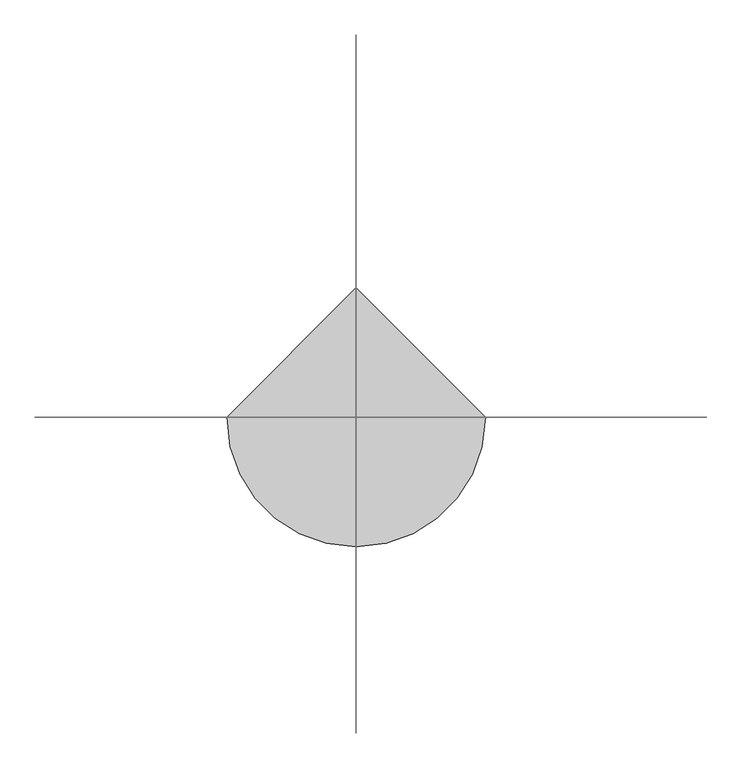
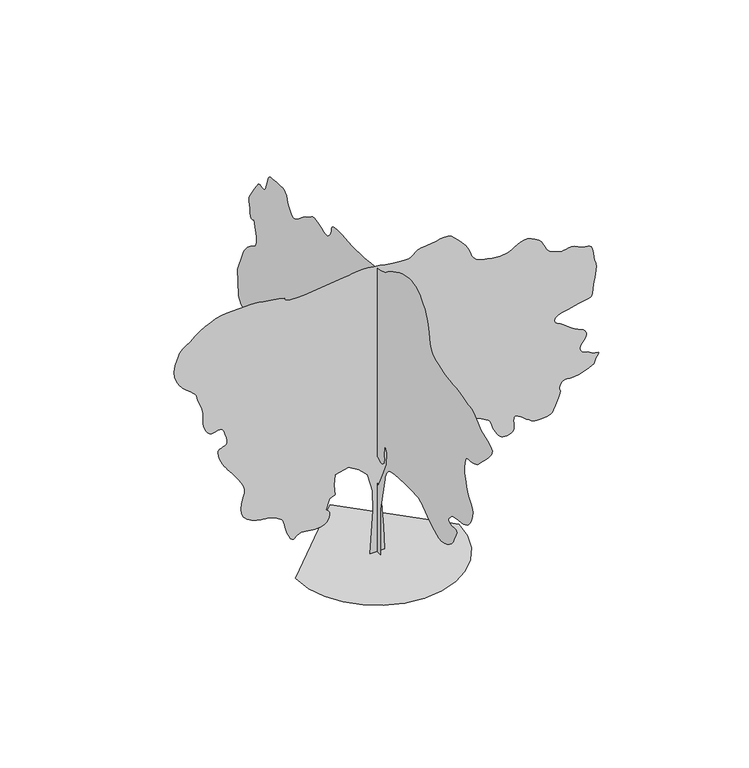
"""IFC4 building model written with IfcOpenShell, lengths in millimetres: geographic element geometry, RPC 木 - 落葉樹 : リンゴの木 - 6.0 メートル."""

from ifc_helpers import new_model, si_unit, origin, place, context, project, spatial, triangles, source, transform, mapped, element, save


def geographic_element_a7a636f8(model_context):
    return source(origin(), model_context, "Body", "Tessellation", [
        triangles([(-6.51e-05, -105.0228319, 0.0074776), (-6.15e-05, 138.9131143, 0.0074703), (-4.84e-05, 99.8833291, 458.6078719), (-3.14e-05, 129.1556067, 1014.7807915), (-1.8e-05, 226.7299288, 1414.8361691), (-8.5e-06, 392.6053236, 1649.0138809), (-1.1e-06, 577.9979682, 1805.1340027), (2.6e-06, 753.6305981, 1844.161417), (3.5e-06, 948.7807503, 1775.8613708), (1.5e-06, 1007.3257959, 1678.2863674), (-4e-06, 890.2357046, 1551.4387321), (-8.4e-06, 929.2657351, 1385.5635372), (-1.44e-05, 1153.685903, 1073.3258371), (-1.47e-05, 1543.9836639, 868.4182137), (-8.5e-06, 2109.9142365, 790.3606236), (7.6e-06, 2451.4244957, 1161.1408985), (2.53e-05, 2802.702182, 1580.7112186), (3.2e-05, 3349.1025513, 1531.9237896), (3.84e-05, 3544.2528488, 1649.0138809), (4.53e-05, 3534.5028625, 1883.1914474), (4.5e-05, 3358.8778267, 1961.2515083), (4.95e-05, 3232.0277206, 2175.9142776), (5.43e-05, 3534.5028625, 2185.6716763), (5.98e-05, 4139.453437, 2068.584201), (6.19e-05, 4208.0283211, 2104.1717091), (6.39e-05, 4273.9283684, 2140.0141434), (6.59e-05, 4334.553447, 2176.3691917), (6.78e-05, 4387.2284294, 2213.4942513), (6.96e-05, 4429.328476, 2251.6417774), (7.12e-05, 4458.2034576, 2291.0693127), (7.26e-05, 4471.2035362, 2332.0343994), (8.79e-05, 4500.4784935, 2829.6522812), (9.79e-05, 4334.6034439, 3249.2275429), (9.86e-05, 4317.5033249, 3282.3275574), (9.94e-05, 4292.2284142, 3321.5527794), (0.0001002, 4260.1033401, 3364.7027618), (0.000101, 4222.5283081, 3409.5526405), (0.0001017, 4180.8532356, 3453.9028404), (0.0001023, 4136.4533295, 3495.527916), (0.0001027, 4090.6782166, 3532.2027122), (0.0001029, 4046.5782921, 3560.9279938), (0.0001029, 4006.7531067, 3582.8278198), (0.000103, 3971.8782005, 3601.8278229), (0.0001031, 3942.6282417, 3621.8527634), (0.0001036, 3919.7031876, 3646.8529816), (0.0001043, 3903.7779968, 3680.7029503), (0.0001056, 3895.5282097, 3727.3530098), (0.0001072, 3894.4779831, 3782.2781456), (0.0001089, 3899.0529945, 3838.2279282), (0.0001108, 3908.3280098, 3895.0532387), (0.0001127, 3921.3530869, 3952.5282188), (0.0001147, 3937.2032822, 4010.528167), (0.0001167, 3954.9280724, 4068.8783844), (0.0001187, 3973.5780968, 4127.4033005), (0.0001184, 3998.5533165, 4107.2783661), (0.0001184, 4022.8532867, 4091.9531387), (0.0001185, 4045.7783409, 4086.1782005), (0.0001191, 4066.6532295, 4094.7532585), (0.0001202, 4084.8032845, 4122.4283134), (0.0001219, 4099.5532562, 4174.003363), (0.0001245, 4110.1781891, 4254.2534065), (0.000127, 4120.6784203, 4333.2285278), (0.0001287, 4132.0283089, 4385.4035408), (0.0001299, 4139.1281662, 4422.2036201), (0.0001309, 4136.8033081, 4455.0786484), (0.0001318, 4120.0031708, 4495.478508), (0.0001331, 4083.5533607, 4554.8286644), (0.0001348, 4022.3783157, 4644.5537109), (0.0001367, 3956.5782623, 4741.1289207), (0.0001382, 3906.9780922, 4815.003772), (0.0001392, 3869.5280525, 4868.5789902), (0.0001398, 3840.0781059, 4904.2041412), (0.0001401, 3814.5529198, 4924.3290756), (0.0001399, 3788.8780334, 4931.3042313), (0.0001393, 3758.9281174, 4927.5038818), (0.0001386, 3727.67799, 4918.0288788), (0.0001379, 3700.2029228, 4909.0788437), (0.0001374, 3675.45298, 4904.7291092), (0.0001372, 3652.4029335, 4909.0788437), (0.0001374, 3630.0528442, 4926.2289597), (0.000138, 3607.3527763, 4960.2792068), (0.0001393, 3583.2777924, 5015.3287537), (0.0001409, 3562.2279144, 5079.6288986), (0.0001424, 3546.3027237, 5137.7538391), (0.0001437, 3531.0527824, 5188.4042358), (0.0001447, 3512.0527794, 5230.1540131), (0.0001452, 3484.8526955, 5261.6794144), (0.0001452, 3445.0278008, 5281.604361), (0.0001446, 3388.1277855, 5288.5295197), (0.0001436, 3319.3276245, 5291.5793335), (0.0001428, 3248.6275795, 5298.5544891), (0.000142, 3178.9774704, 5306.2040222), (0.0001411, 3113.2274139, 5311.3042923), (0.0001402, 3054.3025223, 5310.5793365), (0.0001392, 3005.1273262, 5300.8293503), (0.000138, 2968.5772316, 5278.778952), (0.0001369, 2944.7272339, 5253.1543533), (0.0001361, 2929.602285, 5232.6294434), (0.0001354, 2919.9272942, 5214.0044174), (0.0001347, 2912.4774582, 5194.003894), (0.0001338, 2904.0023941, 5169.4042328), (0.0001326, 2891.2523003, 5136.9288895), (0.000131, 2871.0023735, 5093.3792221), (0.0001292, 2844.6522377, 5045.379245), (0.0001275, 2815.5772682, 5003.1539154), (0.000126, 2783.4271957, 4968.9542587), (0.0001248, 2747.8773308, 4945.0039764), (0.0001238, 2708.5521149, 4933.504097), (0.0001233, 2665.1521477, 4936.7039017), (0.0001232, 2617.3021614, 4956.7788391), (0.0001234, 2569.6771614, 4988.2542435), (0.0001238, 2525.4769524, 5023.3038483), (0.0001243, 2482.1194244, 5060.7288895), (0.0001247, 2437.0593842, 5099.3538574), (0.0001252, 2387.7318718, 5138.0038239), (0.0001254, 2331.5768692, 5175.4288651), (0.0001255, 2266.0343582, 5210.4790512), (0.0001256, 2205.0142456, 5244.5542969), (0.0001259, 2159.0142918, 5277.6040237), (0.0001262, 2120.3541515, 5306.2290207), (0.0001262, 2081.3542065, 5327.0044968), (0.0001258, 2034.3291698, 5336.5044983), (0.0001247, 1971.6040741, 5331.3292328), (0.0001227, 1885.4940685, 5308.0544907), (0.0001205, 1797.391452, 5276.8540695), (0.0001188, 1730.2863911, 5251.9544266), (0.0001175, 1678.8813892, 5236.1042313), (0.0001168, 1637.8888332, 5232.0288986), (0.0001166, 1602.0163136, 5242.4794235), (0.0001169, 1565.9737461, 5270.1544785), (0.0001177, 1524.4687214, 5317.8044769), (0.0001188, 1490.9861721, 5373.8045471), (0.0001201, 1475.2561729, 5423.9793915), (0.0001212, 1466.3511932, 5467.3296524), (0.0001221, 1453.3511147, 5502.8292297), (0.0001225, 1425.3286972, 5529.4543488), (0.0001222, 1371.366148, 5546.1794907), (0.000121, 1280.5334656, 5551.979718), (0.0001195, 1182.4759335, 5550.8792038), (0.0001183, 1108.9958982, 5547.8793869), (0.0001174, 1052.4133781, 5543.5296524), (0.0001165, 1005.0483187, 5538.3293884), (0.0001156, 959.220738, 5532.7791458), (0.0001147, 907.2482563, 5527.4044739), (0.0001136, 841.4482029, 5522.7041794), (0.0001125, 772.3506037, 5519.7043625), (0.0001115, 711.6155754, 5518.9044113), (0.0001107, 653.2705175, 5520.154335), (0.0001099, 591.3404677, 5523.2791443), (0.000109, 519.8504273, 5528.1294296), (0.0001078, 432.8303392, 5534.5046219), (0.0001065, 324.3052774, 5542.2291504), (0.000105, 203.687658, 5552.8796631), (0.0001037, 86.9965703, 5567.6043457), (0.0001026, -21.8426915, 5585.7544006), (0.0001018, -118.9050968, 5606.6292892), (0.0001012, -200.2644113, 5629.5546341), (0.0001011, -261.9952181, 5653.8543137), (0.0001012, -300.1702317, 5678.8295334), (0.0001016, -342.4727732, 5713.0297714), (0.000102, -413.9603428, 5761.2297363), (0.0001023, -506.7854181, 5817.0798157), (0.0001024, -613.0929554, 5874.3298096), (0.0001023, -725.0330704, 5926.6045258), (0.0001019, -834.75319, 5967.6299286), (0.0001011, -934.4057556, 5991.07966), (0.0001, -1022.9033335, 5999.8047089), (9.88e-05, -1104.7484104, 6000.0046967), (9.74e-05, -1180.4459702, 5990.3047073), (9.57e-05, -1250.5110249, 5969.3298248), (9.38e-05, -1315.4560432, 5935.7295502), (9.14e-05, -1375.7936394, 5888.1545471), (8.87e-05, -1432.0336658, 5825.2049011), (8.63e-05, -1478.7161362, 5768.8048553), (8.48e-05, -1512.7687088, 5733.7546692), (8.36e-05, -1538.2837212, 5707.9295013), (8.25e-05, -1559.3636845, 5679.2045105), (8.09e-05, -1580.1012268, 5635.454274), (7.84e-05, -1604.5962433, 5564.5545319), (7.46e-05, -1636.941362, 5454.4042786), (7.05e-05, -1667.1512913, 5330.3292938), (6.7e-05, -1688.656374, 5223.97939), (6.39e-05, -1710.6739254, 5132.8541382), (6.11e-05, -1742.4214062, 5054.3292801), (5.83e-05, -1793.1164223, 4985.8788071), (5.53e-05, -1871.9714928, 4924.9540375), (5.19e-05, -1988.2065491, 4868.9789658), (4.87e-05, -2119.0091755, 4825.5040031), (4.62e-05, -2237.6917568, 4799.6038399), (4.41e-05, -2347.6668755, 4784.9788605), (4.22e-05, -2452.3543808, 4775.3288681), (4.04e-05, -2555.1521759, 4764.2786705), (3.83e-05, -2659.5022018, 4745.5539413), (3.57e-05, -2768.8022163, 4712.8539024), (3.33e-05, -2866.4523605, 4683.5786545), (3.19e-05, -2939.5522591, 4672.2287659), (3.09e-05, -2996.927536, 4668.05373), (2.99e-05, -3047.4773575, 4660.2786232), (2.85e-05, -3100.0773445, 4638.1788094), (2.61e-05, -3163.6025368, 4590.9787834), (2.24e-05, -3246.9276833, 4507.9536186), (1.83e-05, -3354.9527756, 4422.0536293), (1.48e-05, -3474.4277504, 4364.503363), (1.18e-05, -3586.9278603, 4321.8033531), (9.3e-06, -3673.9780701, 4280.47855), (7e-06, -3717.153051, 4227.0283241), (5e-06, -3698.0280556, 4147.9782074), (2.9e-06, -3598.177755, 4029.8281517), (1.1e-06, -3473.4528099, 3906.2781349), (-3e-07, -3385.2276718, 3815.6781418), (-1.3e-06, -3323.4776619, 3751.5279877), (-1.9e-06, -3278.1025246, 3707.3530678), (-2.2e-06, -3239.0275841, 3676.6529068), (-2.3e-06, -3196.2275803, 3652.9528999), (-2.1e-06, -3139.5775497, 3629.777861), (-1.7e-06, -3075.1774109, 3613.37799), (-9e-07, -3016.2275208, 3608.6029907), (-2e-07, -2963.4272552, 3606.7278145), (2e-07, -2917.4774437, 3599.0529922), (2e-07, -2879.0021759, 3576.8528938), (-7e-07, -2848.7272797, 3531.452758), (-2.7e-06, -2827.3521309, 3454.1278267), (-5.1e-06, -2815.7522575, 3369.9277336), (-7e-06, -2813.3521133, 3305.0276253), (-8.6e-06, -2818.6523712, 3252.4026398), (-1.02e-05, -2830.0772552, 3205.052623), (-1.19e-05, -2846.1271477, 3156.0024193), (-1.39e-05, -2865.2274353, 3098.2524559), (-1.64e-05, -2885.9023361, 3024.8022881), (-1.92e-05, -2914.627327, 2946.6774055), (-2.18e-05, -2954.4522217, 2877.5772629), (-2.43e-05, -2998.5524368, 2814.6273262), (-2.67e-05, -3040.0775185, 2754.9021927), (-2.9e-05, -3072.2275909, 2695.5270378), (-3.11e-05, -3088.152491, 2633.6020386), (-3.3e-05, -3081.052343, 2566.2020828), (-3.46e-05, -3060.4274391, 2500.277037), (-3.6e-05, -3039.1022873, 2443.7194427), (-3.71e-05, -3015.2522896, 2395.18694), (-3.79e-05, -2986.9272743, 2353.3118797), (-3.85e-05, -2952.3273514, 2316.7293743), (-3.88e-05, -2909.5023491, 2284.0717747), (-3.89e-05, -2856.6273788, 2253.9743385), (-3.87e-05, -2791.7272705, 2230.5618141), (-3.8e-05, -2717.452153, 2216.0268002), (-3.71e-05, -2638.7520149, 2206.0967377), (-3.62e-05, -2560.5271385, 2196.5117123), (-3.56e-05, -2487.799601, 2182.9993103), (-3.53e-05, -2425.47201, 2161.2942398), (-3.56e-05, -2378.5043827, 2127.129174), (-3.62e-05, -2345.7043499, 2089.8041267), (-3.68e-05, -2322.8042942, 2060.3341232), (-3.73e-05, -2310.1443111, 2037.0066227), (-3.78e-05, -2308.0692924, 2018.1191128), (-3.84e-05, -2316.9168629, 2001.9616688), (-3.92e-05, -2337.029298, 1986.8265461), (-4.01e-05, -2368.7468388, 1971.0090523), (-4.1e-05, -2411.2468609, 1962.5040482), (-4.16e-05, -2459.0394379, 1965.0915356), (-4.21e-05, -2505.4770103, 1970.754126), (-4.27e-05, -2543.876992, 1971.4641117), (-4.34e-05, -2567.6019974, 1959.2041042), (-4.44e-05, -2569.9771431, 1925.949012), (-4.59e-05, -2544.3769615, 1863.6765049), (-4.75e-05, -2509.7520401, 1792.5014889), (-4.89e-05, -2484.8695473, 1735.1513557), (-4.99e-05, -2462.7095627, 1687.5312973), (-5.08e-05, -2436.2819607, 1645.5437439), (-5.14e-05, -2398.5893486, 1605.0912712), (-5.19e-05, -2342.631863, 1562.0787804), (-5.22e-05, -2261.4142914, 1512.4087017), (-5.2e-05, -2169.1316975, 1473.3237328), (-5.1e-05, -2083.5066914, 1461.3762062), (-4.95e-05, -2002.8290577, 1471.4462311), (-4.76e-05, -1925.3965748, 1498.4137711), (-4.53e-05, -1849.4990273, 1537.1587898), (-4.28e-05, -1773.4289612, 1582.5612511), (-4.02e-05, -1695.4838642, 1629.498793), (-3.77e-05, -1622.0062271, 1676.8063705), (-3.54e-05, -1558.0836754, 1724.7963192), (-3.31e-05, -1500.136195, 1770.5689613), (-3.11e-05, -1444.578685, 1811.2214218), (-2.93e-05, -1387.8260445, 1843.8489361), (-2.77e-05, -1326.2960793, 1865.5564774), (-2.64e-05, -1256.4010723, 1873.4340488), (-2.5e-05, -1159.1384045, 1874.2889385), (-2.3e-05, -1027.910804, 1875.4840691), (-2.07e-05, -877.7382116, 1874.971455), (-1.86e-05, -723.6380974, 1870.7039829), (-1.67e-05, -580.6329818, 1860.6339581), (-1.55e-05, -463.7428782, 1842.7115055), (-1.52e-05, -387.9878002, 1814.8914013), (-1.57e-05, -343.2127716, 1776.8839828), (-1.66e-05, -308.1652379, 1730.6863667), (-1.77e-05, -281.2252217, 1677.6614056), (-1.92e-05, -260.7727092, 1619.1738419), (-2.08e-05, -245.1829449, 1556.5887085), (-2.26e-05, -232.8366782, 1491.2736546), (-2.44e-05, -222.1121693, 1424.5935677), (-3.85e-05, -114.7803395, 897.6907001), (-2.01e-05, -26.9632706, 1297.7460777), (-1.3e-05, -173.3248856, 1609.9838505), (-6.5e-06, -300.1727388, 1892.9489914), (2e-07, -319.6852469, 2127.129174), (4.7e-06, -251.3852008, 2244.2167946), (-4e-07, -222.1119331, 2058.8266571), (-1.7e-06, -228.0859325, 2017.1790539), (-3e-06, -232.2679447, 1976.5565334), (-4.1e-06, -232.865183, 1937.9815624), (-5.1e-06, -228.0859325, 1902.4790783), (-5.9e-06, -216.1379155, 1871.0740185), (-6.4e-06, -195.2293988, 1844.788995), (-6.5e-06, -163.5673779, 1824.6489452), (-6.1e-06, -127.1833524, 1819.4714996), (-5.2e-06, -93.5303284, 1831.0189053), (-4.2e-06, -62.949051, 1849.7389835), (-3.3e-06, -35.7820297, 1866.0664753), (-2.9e-06, -12.3698845, 1870.4490566), (-3.1e-06, 6.9458055, 1853.3239391), (-4.3e-06, 21.8237678, 1805.1340027), (-6.1e-06, 32.3777748, 1741.0688725), (-7.7e-06, 39.3472803, 1682.1263947), (-9.3e-06, 43.330036, 1627.4512436), (-1.08e-05, 44.9230347, 1576.1888203), (-1.22e-05, 44.724037, 1527.4862698), (-1.37e-05, 43.330036, 1480.4911732), (-1.51e-05, 41.3385332, 1434.3511116), (137.391859, 0.0003253, 0.0), (-133.3141101, 0.0003334, 0.0), (-73.1573078, 0.0002372, 832.1731876), (-83.1833128, 0.0002433, 1223.1935062), (-183.4456522, 0.0001982, 1574.1087147), (-333.8377625, 0.0002049, 1724.5014244), (-534.3604428, 0.0002126, 1844.8164642), (-785.015601, 0.0002192, 1784.6589443), (-805.0681561, 0.0002168, 1584.1363003), (-785.015601, 0.0002134, 1393.6386257), (-885.278231, 0.0002156, 1343.5060753), (-955.4607931, 0.0002149, 1153.0084007), (-936.3432827, 0.0002675, 1139.8859459), (-918.5407356, 0.0002668, 1125.3558735), (-903.3707314, 0.0002661, 1108.0233559), (-892.1456898, 0.0002654, 1086.4808481), (-886.1831903, 0.0002648, 1059.3258196), (-886.7981964, 0.0002643, 1025.1533415), (-895.3032005, 0.0002639, 982.565752), (-913.9532249, 0.0002639, 940.0632591), (-942.5982788, 0.0002642, 906.5057144), (-978.963283, 0.0002649, 881.0181713), (-1020.7633478, 0.0002659, 862.7181982), (-1065.71838, 0.0002671, 850.7331739), (-1111.553373, 0.0002683, 844.1856812), (-1155.9834372, 0.0002696, 842.1981571), (-1199.4784567, 0.000271, 844.8881819), (-1243.6759769, 0.0002724, 851.4356747), (-1288.0485592, 0.0002738, 859.5631582), (-1332.0685467, 0.0002752, 866.9856703), (-1375.2135876, 0.0002766, 871.4282043), (-1416.9560978, 0.0002778, 870.610667), (-1456.7686386, 0.0002789, 862.2507122), (-1490.9986713, 0.0002796, 844.3906832), (-1518.2137253, 0.0002801, 821.2681847), (-1541.2187164, 0.0002805, 799.9006662), (-1562.8187061, 0.0002809, 787.3031067), (-1585.8236973, 0.0002817, 790.4881594), (-1613.0387512, 0.0002829, 816.475672), (-1647.2663132, 0.0002313, 872.2782251), (-1679.7413658, 0.0002334, 944.3882858), (-1702.0463997, 0.0002351, 1013.3457773), (-1717.508828, 0.0002365, 1077.2133905), (-1729.4639122, 0.0002377, 1134.0684231), (-1741.2438618, 0.0002387, 1181.9784348), (-1756.1814674, 0.0002397, 1219.0134562), (-1777.6064678, 0.0002407, 1243.2460613), (-1804.2939377, 0.0002418, 1262.5659576), (-1833.963929, 0.000243, 1284.8709915), (-1868.368951, 0.0002444, 1308.2261066), (-1909.2639839, 0.000246, 1330.7035137), (-1958.3990662, 0.0002477, 1350.3761501), (-2017.5341194, 0.0002497, 1365.3136105), (-2088.4191822, 0.0002519, 1373.5860706), (-2170.7616852, 0.0002011, 1382.5010788), (-2258.5417923, 0.000204, 1401.9385551), (-2344.9193687, 0.0002071, 1433.8310852), (-2423.054425, 0.0002101, 1480.1036968), (-2486.1043556, 0.0002129, 1542.6862141), (-2527.2271362, 0.0002153, 1623.5087517), (-2539.6019623, 0.0002172, 1724.5014244), (-2528.5270569, 0.0002183, 1822.2489464), (-2508.6771057, 0.0002189, 1897.5490013), (-2487.2420769, 0.0002192, 1958.6416386), (-2471.4293793, 0.0001661, 2013.7690876), (-2468.4170631, 0.0001669, 2071.1791008), (-2485.3994568, 0.0001684, 2139.1117275), (-2529.5769928, 0.000171, 2225.8093426), (-2588.3771828, 0.0001741, 2318.6767845), (-2644.0269836, 0.000177, 2400.3194756), (-2695.8270195, 0.0001796, 2471.7869156), (-2743.0773331, 0.000182, 2534.1270058), (-2785.0520966, 0.0001306, 2588.4271797), (-2821.0522247, 0.0001324, 2635.6772026), (-2850.4021774, 0.0001339, 2676.9770073), (-2878.5522034, 0.0001354, 2723.8270546), (-2908.6274025, 0.0001372, 2782.7522369), (-2936.4274498, 0.000139, 2847.4523575), (-2957.7523109, 0.0001406, 2911.6522179), (-2968.3522453, 0.0001418, 2969.0024963), (-2964.0525078, 0.0001423, 3013.2024147), (-2940.6524826, 0.000142, 3037.927359), (-2905.0023331, 0.0001411, 3050.052491), (-2869.2021927, 0.0001402, 3062.5523094), (-2836.72714, 0.0001395, 3078.1775185), (-2811.1022507, 0.000139, 3099.7773628), (-2795.8023125, 0.000139, 3130.1525436), (-2794.3771088, 0.0001396, 3172.1025993), (-2810.3022995, 0.0001409, 3228.4276497), (-2831.7271545, 8.9e-05, 3286.3526024), (-2846.6774048, 9.02e-05, 3332.2027107), (-2858.4522675, 9.1e-05, 3367.3276016), (-2870.4024101, 9.18e-05, 3393.1777679), (-2885.8523392, 9.25e-05, 3411.1278351), (-2908.17743, 9.33e-05, 3422.5777176), (-2940.6524826, 9.44e-05, 3428.9526192), (-2978.7524826, 9.55e-05, 3427.0527351), (-3016.0025345, 9.65e-05, 3417.4277412), (-3052.7023293, 9.74e-05, 3407.1277885), (-3089.2524239, 9.85e-05, 3403.1027435), (-3125.9775078, 9.97e-05, 3412.4277557), (-3163.2025612, 0.0001012, 3442.1026886), (-3201.3275597, 0.0001032, 3499.1276962), (-3229.5025841, 0.0001051, 3569.6277534), (-3241.3777313, 0.0001065, 3637.1529922), (-3243.9525742, 0.0001076, 3704.8529297), (-3244.2275574, 0.0001086, 3775.9029533), (-3249.2525414, 5.65e-05, 3853.4031647), (-3266.0276802, 5.83e-05, 3940.5780762), (-3301.5775452, 6.09e-05, 4040.5533691), (-3337.877655, 6.33e-05, 4130.928376), (-3357.5276184, 6.48e-05, 4192.7283829), (-3368.4028267, 6.58e-05, 4234.1784691), (-3378.4027977, 6.65e-05, 4263.5284218), (-3395.4276306, 6.74e-05, 4289.0033203), (-3427.3277184, 6.88e-05, 4318.8785316), (-3482.0528664, 7.1e-05, 4361.3785538), (-3552.8529053, 2.06e-05, 4417.8785934), (-3623.6529442, 2.37e-05, 4484.3786041), (-3688.3030678, 2.68e-05, 4561.0535751), (-3740.6780685, 2.96e-05, 4648.0787865), (-3774.6530296, 3.21e-05, 4745.6289368), (-3784.0780357, 3.4e-05, 4853.8540169), (-3762.7778824, 3.51e-05, 4972.9790131), (-3729.8778557, -1.77e-05, 5076.7040771), (-3704.502951, -1.74e-05, 5145.8539261), (-3680.7029503, -1.74e-05, 5191.3290573), (-3652.5279259, -1.78e-05, 5224.0043884), (-3614.0029518, -1.85e-05, 5254.7792542), (-3559.1778099, -1.95e-05, 5294.454158), (-3482.0528664, -2.09e-05, 5353.9790131), (-3391.1775993, -2.26e-05, 5424.8793365), (-3298.9027084, -2.44e-05, 5490.3794083), (-3205.0276245, -2.63e-05, 5548.6543396), (-3109.4273552, -2.84e-05, 5598.0042343), (-3011.8774956, -3.07e-05, 5636.6297836), (-2912.2274734, -3.33e-05, 5662.8293472), (-2810.3022995, -3.62e-05, 5674.8047791), (-2339.0719059, -5.01e-05, 5684.8297485), (-2273.3618179, -5.21e-05, 5682.2043274), (-2197.6542297, -5.44e-05, 5674.854776), (-2113.614156, -3.7e-06, 5663.5293045), (-2022.9115528, -6.6e-06, 5649.0546066), (-1927.2115803, -9.7e-06, 5632.2294708), (-1828.1764915, -1.3e-05, 5613.8044327), (-1727.4763882, -1.63e-05, 5594.6044418), (-1724.3188774, -1.66e-05, 5575.4544479), (-1715.1112999, -1.72e-05, 5557.4543839), (-1693.8014088, -1.8e-05, 5541.7291809), (-1654.3413174, -1.94e-05, 5529.4293503), (-1590.6763081, -2.14e-05, 5521.6792419), (-1496.7561687, -2.42e-05, 5519.6293671), (-1366.5335941, -2.81e-05, 5524.4296555), (-604.5454757, -4.94e-05, 5614.6543808), (-529.8304141, -5.15e-05, 5621.554541), (-464.7628741, 1e-07, 5631.7794983), (-403.0278342, -1.6e-06, 5642.554422), (-338.3102729, -3.4e-06, 5651.0294861), (-264.297712, -5.6e-06, 5654.4042801), (-174.6758932, -8.3e-06, 5649.9045547), (-63.1312982, -1.19e-05, 5634.7043198), (53.8502923, -1.57e-05, 5614.4793915), (156.9766284, -1.9e-05, 5596.879303), (248.3524462, -2.19e-05, 5582.1046234), (330.0827591, -2.45e-05, 5570.2791824), (404.2703093, -2.69e-05, 5561.6297104), (473.0203643, -2.9e-05, 5556.304454), (538.4379192, -3.1e-05, 5554.5045639), (593.7429737, -3.25e-05, 5562.8296371), (635.895488, -3.35e-05, 5584.3044891), (672.6080727, -3.41e-05, 5613.6794403), (711.6030762, -3.48e-05, 5645.7042297), (760.5931091, -3.58e-05, 5675.0797623), (827.2981945, -3.75e-05, 5696.5546143), (919.4332684, -4.01e-05, 5704.904686), (1019.3733164, -4.3e-05, 5711.6048584), (1106.3358862, -4.54e-05, 5726.7545151), (1183.3009558, -4.74e-05, 5742.7796997), (1253.2485031, -4.94e-05, 5752.1297104), (1319.1659912, -5.14e-05, 5747.279425), (1384.0286018, -5.37e-05, 5720.6793045), (1450.8211819, -3.2e-06, 5664.7798096), (1514.7787605, -6.1e-06, 5597.4042709), (1569.6162563, -8.6e-06, 5539.5043167), (1616.0337719, -1.07e-05, 5488.254538), (1654.7363514, -1.26e-05, 5440.8795227), (1686.421336, -1.42e-05, 5394.5544434), (1711.7939152, -1.57e-05, 5346.4544724), (1731.5539009, -1.7e-05, 5293.8291962), (1749.3263626, -1.84e-05, 5241.0039322), (1770.606459, -1.97e-05, 5194.1538849), (1798.9013889, -2.12e-05, 5153.0790665), (1837.7189323, 3.06e-05, 5117.6039063), (1890.5690495, 2.85e-05, 5087.6039932), (1960.9566135, 2.61e-05, 5062.8287613), (2052.3915848, 2.3e-05, 5043.1537994), (2147.2741653, 2e-05, 5028.9540848), (2227.0742363, 1.75e-05, 5020.3540283), (2293.8969017, 1.55e-05, 5016.8542419), (2349.8443588, 1.38e-05, 5017.9041779), (2397.0244732, 1.25e-05, 5023.0038666), (2437.5369713, 1.14e-05, 5031.5789246), (2473.4920441, 1.05e-05, 5043.1537994), (2512.0269012, 9.7e-06, 5063.479303), (2558.2519867, 8.7e-06, 5093.9791855), (2611.3522339, 7.6e-06, 5127.6038773), (2670.3771194, 6.3e-06, 5157.4043839), (2734.5272736, 4.7e-06, 5176.304393), (2802.8521729, 2.7e-06, 5177.3293304), (2874.5271584, 2e-07, 5153.4540436), (2937.3023964, -2.2e-06, 5120.2293274), (2982.5272522, -3.9e-06, 5095.0541199), (3014.7523201, -5.2e-06, 5073.7292587), (3038.5773193, -6.2e-06, 5052.0788361), (3058.5525536, -7.2e-06, 5025.854274), (3079.2024559, -8.3e-06, 4990.8790833), (3105.1276176, -9.8e-06, 4942.9041046), (3132.7273865, 4.2e-05, 4892.8036743), (3157.7026062, 4.07e-05, 4852.7037964), (3183.5274834, 3.94e-05, 4820.3037392), (3213.7526733, 3.81e-05, 4793.3539307), (3251.8776718, 3.66e-05, 4769.5539299), (3301.4025558, 3.48e-05, 4746.6538742), (3365.8276932, 3.25e-05, 4722.3289055), (3431.1277771, 3.03e-05, 4707.5036476), (3484.3277275, 2.88e-05, 4709.3538254), (3530.502816, 2.76e-05, 4719.9537598), (3574.7527313, 2.64e-05, 4731.4539299), (3622.1780342, 2.51e-05, 4735.9286568), (3677.8278351, 2.33e-05, 4725.4787132), (3746.8029854, 2.07e-05, 4692.2537064), (3818.1279922, 1.81e-05, 4658.4537346), (3877.8781242, 1.61e-05, 4644.1287369), (3926.7530479, 1.45e-05, 4638.053817), (3965.453302, 1.32e-05, 4629.003788), (3994.7032608, 1.2e-05, 4605.7287552), (4015.1531754, 6.41e-05, 4557.0285301), (4027.5532906, 6.24e-05, 4471.6785072), (4039.2031609, 6.08e-05, 4384.4785973), (4054.5533867, 5.95e-05, 4327.8035683), (4069.9033218, 5.84e-05, 4286.7284592), (4081.5781906, 5.75e-05, 4246.3533073), (4085.8532204, 5.65e-05, 4191.7784409), (4079.1033417, 5.55e-05, 4108.1033157), (4057.628199, 5.42e-05, 3980.3782631), (4035.5280945, 0.0001063, 3847.1779633), (4024.4781876, 0.0001052, 3752.0279572), (4017.103347, 0.0001045, 3687.5778214), (4006.0531494, 0.0001042, 3646.453006), (3983.9530449, 0.0001045, 3621.2777985), (3943.4531914, 0.0001054, 3604.7279366), (3877.1531685, 0.0001072, 3589.3780014), (3783.9280449, 0.0001097, 3571.4279343), (3675.2779907, 0.0001126, 3551.3777046), (3562.7778809, 0.0001156, 3528.3279488), (3457.9778824, 0.0001183, 3501.452845), (3372.477578, 0.0001204, 3469.8277405), (3317.8527145, 0.0001215, 3432.5776886), (3305.6525871, 0.0001212, 3388.8527412), (3318.4276794, 0.0001203, 3351.9776665), (3332.9526649, 0.0001195, 3330.9027901), (3352.2276512, 0.0001188, 3318.0777008), (3379.2027489, 0.0001178, 3305.9525688), (3416.8777748, 0.0001164, 3286.9775642), (3468.2528366, 0.0001143, 3253.627565), (3536.2527557, 0.0001115, 3198.3524506), (3611.5028137, 0.0001084, 3139.7525391), (3681.477903, 0.0001057, 3097.8024834), (3744.6281181, 0.0001033, 3067.0773239), (3799.3529755, 0.0001547, 3042.1273933), (3844.053154, 0.000153, 3017.5524399), (3877.2031654, 0.0001516, 2987.877507), (3897.2031075, 0.0001504, 2947.702343), (3897.9280632, 0.0001497, 2900.4773186), (3879.7280113, 0.0001495, 2853.6272713), (3850.6530418, 0.0001497, 2807.4771812), (3818.7529541, 0.00015, 2762.3773178), (3792.1281258, 0.0001501, 2718.6770782), (3778.8280655, 0.0001499, 2676.7270226), (3786.9281525, 0.0001491, 2636.8771294), (3809.6279297, 0.0001479, 2605.4770111), (3834.8031372, 0.0001469, 2585.8520462), (3862.4281952, 0.0001459, 2573.7522034), (3892.5031036, 0.0001448, 2564.9771576), (3925.0281532, 0.0001437, 2555.3271652), (3960.0280518, 0.0001425, 2540.6019012), (3997.4780914, 0.000141, 2516.5769142), (4036.1783455, 0.0001395, 2494.674472), (4072.603157, 0.0001383, 2485.0593613), (4103.2283226, 0.0001373, 2481.5793411), (4124.5531837, 0.0001366, 2478.1019371), (4133.1032433, 0.0001362, 2468.4845009), (4125.3284271, 0.0001895, 2446.5919418), (4097.7283676, 0.0001897, 2406.2819023), (4070.2033035, 0.0001899, 2361.9969601), (4057.9281807, 0.0001898, 2329.461882), (4050.3783508, 0.0001896, 2304.4693668), (4037.0532921, 0.0001897, 2282.8093517), (4007.403067, 0.0001903, 2260.2742447), (3950.9280258, 0.0001915, 2232.649332), (3857.1032295, 0.0001938, 2195.731818), (3751.1030136, 0.0001965, 2165.9741867), (3663.5278358, 0.000199, 2156.5616798), (3591.9278458, 0.0002011, 2158.3742146), (3533.8029053, 0.0002029, 2162.291708), (3486.7528702, 0.0002043, 2159.1942226), (3448.2778931, 0.0002051, 2139.9592049), (3415.9528313, 0.0002054, 2095.4691879), (3396.9028313, 0.0002053, 2048.9641777), (3394.8526657, 0.000205, 2022.9766651), (3402.2777939, 0.0002045, 2007.3391022), (3411.6278046, 0.000204, 1991.8765285), (3415.3778664, 0.0002035, 1966.4166), (3405.9528603, 0.0002031, 1920.7865364), (3375.8526627, 0.0002029, 1844.8164642), (3339.8025375, 0.0002027, 1759.2289558), (3313.4026955, 0.0002024, 1690.476321), (3290.3526489, 0.0002023, 1636.9838013), (3264.3024948, 0.0002025, 1597.1712605), (3228.9526176, 0.0002032, 1569.4613239), (3178.0025299, 0.0002044, 1552.2737103), (3105.1276176, 0.0002065, 1544.0311901), (3032.1274223, 0.0002086, 1540.6111954), (2980.1523972, 0.0002101, 1539.996262), (2942.0273987, 0.0002113, 1543.7687061), (2910.5772835, 0.0002124, 1553.5012516), (2878.6022003, 0.0002136, 1570.7762146), (2838.902298, 0.0002152, 1597.1712605), (2784.3021423, 0.0002174, 1634.2663799), (2725.2272598, 0.0002198, 1675.6263554), (2676.327047, 0.0002218, 1712.2539162), (2636.7271385, 0.0002234, 1741.8638821), (2605.5270081, 0.0002246, 1762.1813919), (2581.8769981, 0.0002254, 1770.9214108), (2564.9021622, 0.0002259, 1765.8038452), (2553.7019737, 0.0002259, 1744.5538342), (2547.3770691, 0.0002257, 1717.2514309), (2544.9269279, 0.0002254, 1694.3364052), (2545.2769066, 0.0002251, 1674.0488354), (2547.3770691, 0.0002247, 1654.6388283), (2550.2018967, 0.0002244, 1634.3538746), (2552.6520378, 0.0002239, 1611.4362328), (2553.7019737, 0.0002235, 1584.1363003), (2552.2770607, 0.0002231, 1554.2312943), (2547.1520828, 0.0002228, 1525.3811657), (2537.1271133, 0.0002227, 1498.6361412), (2520.9519379, 0.0002229, 1475.0461567), (2497.4295364, 0.0002233, 1455.666235), (2465.3044624, 0.000224, 1441.5461666), (2423.3594936, 0.0002251, 1433.7435905), (2380.6244568, 0.0002264, 1432.0761051), (2345.4293667, 0.0002275, 1436.3736626), (2315.4968914, 0.0002286, 1447.6861988), (2288.5467922, 0.0002297, 1467.0661205), (2262.2967957, 0.0002309, 1495.5661251), (2234.4692791, 0.0002323, 1534.2387646), (2202.7842945, 0.000234, 1584.1363003), (2173.4642818, 0.0002356, 1638.6213467), (2152.3892601, 0.0001837, 1689.7763638), (2136.7516972, 0.0001848, 1736.7213181), (2123.7442062, 0.0001858, 1778.5789375), (2110.561726, 0.0001868, 1814.4739849), (2094.3967243, 0.0001877, 1843.5290428), (2072.4441399, 0.0001886, 1864.8690193), (2041.9866966, 0.0001898, 1883.516573), (2003.1091278, 0.0001913, 1904.796524), (1957.2165802, 0.000193, 1928.2690739), (1905.7115845, 0.0001949, 1953.4966038), (1849.996526, 0.000197, 1980.0365536), (1791.4764061, 0.0001991, 2007.4565369), (1731.5539009, 0.0002013, 2035.3141388), (1390.663662, 0.0002115, 2035.3141388), (1200.1659874, 0.0002139, 1814.7364689), (1195.6959841, 0.0002136, 1784.6589443), (1190.1709579, 0.0002133, 1754.578949), (1182.5409731, 0.0002131, 1724.5014244), (1171.7559483, 0.0002129, 1694.4238998), (1156.7583899, 0.0002129, 1664.3437592), (1136.5033762, 0.0002131, 1634.2663799), (1109.9308702, 0.0002134, 1604.1888554), (1086.2834038, 0.0002138, 1578.7562508), (1071.7558748, 0.0002139, 1561.5687824), (1060.7358353, 0.0002141, 1551.0461689), (1047.610837, 0.0002144, 1545.6087101), (1026.7682865, 0.000215, 1543.6787407), (992.5982792, 0.000216, 1543.6787407), (939.4857508, 0.0002176, 1544.0311901), (873.0156801, 0.0002196, 1546.8661915), (804.2656614, 0.0002218, 1554.4362236), (735.8656214, 0.000224, 1565.3387558), (670.4455593, 0.0002262, 1578.1712574), (610.6404888, 0.0002281, 1591.5313431), (559.0754313, 0.0002299, 1604.0112499), (518.3879076, 0.0002312, 1614.2138248), (483.4279049, 0.0002324, 1624.5613037), (447.4153502, 0.0002337, 1638.0662933), (410.5253417, 0.000235, 1654.201355), (372.9353033, 0.0002364, 1672.4413754), (334.8177535, 0.0001845, 1692.2589157), (296.3502432, 0.0001859, 1713.1313335), (257.7052002, 0.0001874, 1734.5288647), (77.2350658, 0.0002405, 1353.5335155), (67.2090517, 0.0002365, 1062.7733562), (117.3398399, 0.0002792, 451.1778749), (-1522.7162121, 1.1e-06, 0.0098235), (-1482.4612564, -348.9052657, 0.0098339), (-1367.8136032, -669.3205553, 0.0098435), (-1187.9534334, -952.0632534, 0.0098519), (-952.0632534, -1187.9534334, 0.0098589), (-669.3205553, -1367.8136032, 0.0098643), (-348.9052657, -1482.4612564, 0.0098677), (6.66e-05, -1522.7162121, 0.0098689), (348.9052657, -1482.4612564, 0.0098677), (669.3205553, -1367.8136032, 0.0098643), (952.0632534, -1187.9534334, 0.0098589), (1187.9534334, -952.0632534, 0.0098519), (1367.8136032, -669.3205553, 0.0098435), (1482.4612564, -348.9052657, 0.0098339), (1522.7162121, 0.0001238, 0.0098235), (-0.0001997, 1522.7162121, 0.0097782)], [[300, 1, 301], [299, 300, 301], [299, 301, 302], [298, 299, 302], [297, 298, 302], [296, 297, 302], [296, 302, 303], [295, 296, 303], [294, 295, 303], [293, 294, 303], [292, 293, 303], [1, 2, 3], [301, 1, 3], [301, 3, 4], [301, 4, 5], [327, 301, 5], [326, 327, 5], [326, 5, 6], [325, 326, 6], [324, 325, 6], [323, 324, 6], [322, 323, 6], [321, 322, 6], [320, 321, 6], [19, 20, 21], [18, 19, 21], [17, 18, 21], [17, 21, 22], [320, 6, 7], [319, 320, 7], [291, 292, 303], [291, 303, 304], [290, 291, 304], [261, 262, 263], [260, 261, 263], [260, 263, 264], [259, 260, 264], [259, 264, 265], [258, 259, 265], [10, 11, 12], [14, 15, 16], [258, 265, 266], [257, 258, 266], [205, 206, 207], [204, 205, 207], [204, 207, 208], [203, 204, 208], [203, 208, 209], [202, 203, 209], [202, 209, 210], [257, 266, 267], [10, 12, 13], [257, 267, 268], [257, 268, 269], [256, 257, 269], [256, 269, 270], [256, 270, 271], [255, 256, 271], [255, 271, 272], [255, 272, 273], [255, 273, 274], [255, 274, 275], [255, 275, 276], [255, 276, 277], [254, 255, 277], [254, 277, 278], [254, 278, 279], [254, 279, 280], [253, 254, 280], [253, 280, 281], [253, 281, 282], [289, 290, 304], [10, 13, 14], [10, 14, 16], [10, 16, 17], [10, 17, 22], [9, 10, 22], [201, 202, 210], [201, 210, 211], [201, 211, 212], [201, 212, 213], [201, 213, 214], [201, 214, 215], [201, 215, 216], [201, 216, 217], [201, 217, 218], [201, 218, 219], [200, 201, 219], [199, 200, 219], [198, 199, 219], [197, 198, 219], [196, 197, 219], [195, 196, 219], [194, 195, 219], [194, 219, 220], [193, 194, 220], [192, 193, 220], [191, 192, 220], [190, 191, 220], [189, 190, 220], [189, 220, 221], [188, 189, 221], [252, 253, 282], [252, 282, 283], [188, 221, 222], [187, 188, 222], [251, 252, 283], [187, 222, 223], [23, 24, 25], [318, 319, 7], [56, 57, 58], [56, 58, 59], [55, 56, 59], [55, 59, 60], [54, 55, 60], [54, 60, 61], [54, 61, 62], [23, 25, 26], [186, 187, 223], [23, 26, 27], [23, 27, 28], [23, 28, 29], [23, 29, 30], [23, 30, 31], [23, 31, 32], [23, 32, 33], [23, 33, 34], [23, 34, 35], [23, 35, 36], [23, 36, 37], [23, 37, 38], [23, 38, 39], [23, 39, 40], [23, 40, 41], [23, 41, 42], [23, 42, 43], [23, 43, 44], [22, 23, 44], [22, 44, 45], [9, 22, 45], [9, 45, 46], [9, 46, 47], [9, 47, 48], [8, 9, 48], [8, 48, 49], [8, 49, 50], [8, 50, 51], [8, 51, 52], [8, 52, 53], [8, 53, 54], [250, 251, 283], [250, 283, 284], [288, 289, 304], [288, 304, 305], [186, 223, 224], [287, 288, 305], [313, 314, 315], [312, 313, 315], [311, 312, 315], [310, 311, 315], [310, 315, 316], [309, 310, 316], [308, 309, 316], [308, 316, 317], [307, 308, 317], [306, 307, 317], [306, 317, 318], [305, 306, 318], [305, 318, 7], [305, 7, 8], [305, 8, 54], [305, 54, 62], [305, 62, 63], [305, 63, 64], [305, 64, 65], [305, 65, 66], [305, 66, 67], [305, 67, 68], [305, 68, 69], [305, 69, 70], [305, 70, 71], [305, 71, 72], [305, 72, 73], [305, 73, 74], [305, 74, 75], [305, 75, 76], [305, 76, 77], [305, 77, 78], [305, 78, 79], [305, 79, 80], [305, 80, 81], [305, 81, 82], [305, 82, 83], [305, 83, 84], [305, 84, 85], [305, 85, 86], [305, 86, 87], [305, 87, 88], [305, 88, 89], [305, 89, 90], [305, 90, 91], [305, 91, 92], [134, 135, 136], [134, 136, 137], [133, 134, 137], [133, 137, 138], [132, 133, 138], [132, 138, 139], [132, 139, 140], [131, 132, 140], [131, 140, 141], [131, 141, 142], [131, 142, 143], [130, 131, 143], [130, 143, 144], [130, 144, 145], [286, 287, 305], [186, 224, 225], [185, 186, 225], [249, 250, 284], [130, 145, 146], [285, 286, 305], [249, 284, 285], [249, 285, 305], [248, 249, 305], [234, 235, 236], [233, 234, 236], [233, 236, 237], [232, 233, 237], [232, 237, 238], [232, 238, 239], [232, 239, 240], [232, 240, 241], [232, 241, 242], [232, 242, 243], [232, 243, 244], [232, 244, 245], [231, 232, 245], [231, 245, 246], [231, 246, 247], [230, 231, 247], [230, 247, 248], [230, 248, 305], [229, 230, 305], [228, 229, 305], [227, 228, 305], [226, 227, 305], [225, 226, 305], [185, 225, 305], [184, 185, 305], [183, 184, 305], [182, 183, 305], [181, 182, 305], [180, 181, 305], [179, 180, 305], [178, 179, 305], [177, 178, 305], [176, 177, 305], [175, 176, 305], [174, 175, 305], [173, 174, 305], [172, 173, 305], [171, 172, 305], [170, 171, 305], [169, 170, 305], [168, 169, 305], [167, 168, 305], [166, 167, 305], [165, 166, 305], [164, 165, 305], [163, 164, 305], [162, 163, 305], [161, 162, 305], [160, 161, 305], [159, 160, 305], [158, 159, 305], [157, 158, 305], [156, 157, 305], [155, 156, 305], [154, 155, 305], [153, 154, 305], [152, 153, 305], [151, 152, 305], [150, 151, 305], [149, 150, 305], [148, 149, 305], [147, 148, 305], [146, 147, 305], [130, 146, 305], [129, 130, 305], [128, 129, 305], [127, 128, 305], [126, 127, 305], [125, 126, 305], [124, 125, 305], [123, 124, 305], [122, 123, 305], [121, 122, 305], [120, 121, 305], [119, 120, 305], [118, 119, 305], [117, 118, 305], [116, 117, 305], [115, 116, 305], [114, 115, 305], [113, 114, 305], [112, 113, 305], [111, 112, 305], [110, 111, 305], [109, 110, 305], [108, 109, 305], [107, 108, 305], [94, 95, 96], [94, 96, 97], [93, 94, 97], [93, 97, 98], [93, 98, 99], [93, 99, 100], [93, 100, 101], [92, 93, 101], [92, 101, 102], [92, 102, 103], [92, 103, 104], [92, 104, 105], [106, 107, 305], [106, 305, 92], [106, 92, 105], [328, 329, 330], [731, 328, 330], [730, 731, 330], [730, 330, 331], [729, 730, 331], [729, 331, 332], [728, 729, 332], [472, 473, 474], [336, 337, 338], [728, 332, 333], [618, 619, 620], [617, 618, 620], [617, 620, 621], [616, 617, 621], [615, 616, 621], [615, 621, 622], [614, 615, 622], [614, 622, 623], [472, 474, 475], [613, 614, 623], [612, 613, 623], [612, 623, 624], [612, 624, 625], [612, 625, 626], [612, 626, 627], [612, 627, 628], [611, 612, 628], [610, 611, 628], [610, 628, 629], [609, 610, 629], [609, 629, 630], [608, 609, 630], [608, 630, 631], [608, 631, 632], [607, 608, 632], [607, 632, 633], [606, 607, 633], [363, 364, 365], [363, 365, 366], [362, 363, 366], [362, 366, 367], [361, 362, 367], [361, 367, 368], [360, 361, 368], [360, 368, 369], [360, 369, 370], [359, 360, 370], [359, 370, 371], [358, 359, 371], [358, 371, 372], [407, 408, 409], [407, 409, 410], [406, 407, 410], [406, 410, 411], [405, 406, 411], [405, 411, 412], [404, 405, 412], [403, 404, 412], [403, 412, 413], [402, 403, 413], [401, 402, 413], [400, 401, 413], [399, 400, 413], [357, 358, 372], [606, 633, 634], [399, 413, 414], [398, 399, 414], [728, 333, 334], [357, 372, 373], [356, 357, 373], [562, 563, 564], [561, 562, 564], [561, 564, 565], [560, 561, 565], [559, 560, 565], [559, 565, 566], [397, 398, 414], [355, 356, 373], [354, 355, 373], [353, 354, 373], [352, 353, 373], [351, 352, 373], [350, 351, 373], [349, 350, 373], [348, 349, 373], [347, 348, 373], [346, 347, 373], [345, 346, 373], [344, 345, 373], [343, 344, 373], [342, 343, 373], [341, 342, 373], [340, 341, 373], [339, 340, 373], [338, 339, 373], [336, 338, 373], [336, 373, 374], [335, 336, 374], [335, 374, 375], [335, 375, 376], [335, 376, 377], [335, 377, 378], [335, 378, 379], [335, 379, 380], [576, 577, 578], [575, 576, 578], [575, 578, 579], [574, 575, 579], [574, 579, 580], [573, 574, 580], [573, 580, 581], [572, 573, 581], [572, 581, 582], [571, 572, 582], [570, 571, 582], [569, 570, 582], [568, 569, 582], [567, 568, 582], [566, 567, 582], [559, 566, 582], [558, 559, 582], [557, 558, 582], [556, 557, 582], [555, 556, 582], [554, 555, 582], [553, 554, 582], [552, 553, 582], [552, 582, 583], [551, 552, 583], [551, 583, 584], [550, 551, 584], [549, 550, 584], [549, 584, 585], [548, 549, 585], [547, 548, 585], [546, 547, 585], [599, 600, 601], [598, 599, 601], [598, 601, 602], [597, 598, 602], [597, 602, 603], [596, 597, 603], [596, 603, 604], [595, 596, 604], [595, 604, 605], [594, 595, 605], [594, 605, 606], [594, 606, 634], [593, 594, 634], [592, 593, 634], [591, 592, 634], [590, 591, 634], [589, 590, 634], [588, 589, 634], [588, 634, 635], [587, 588, 635], [587, 635, 636], [545, 546, 585], [335, 380, 381], [427, 428, 429], [426, 427, 429], [426, 429, 430], [425, 426, 430], [425, 430, 431], [424, 425, 431], [424, 431, 432], [424, 432, 433], [423, 424, 433], [423, 433, 434], [422, 423, 434], [422, 434, 435], [422, 435, 436], [421, 422, 436], [335, 381, 382], [335, 382, 383], [335, 383, 384], [335, 384, 385], [335, 385, 386], [335, 386, 387], [335, 387, 388], [335, 388, 389], [335, 389, 390], [335, 390, 391], [335, 391, 392], [335, 392, 393], [335, 393, 394], [335, 394, 395], [335, 395, 396], [335, 396, 397], [335, 397, 414], [335, 414, 415], [334, 335, 415], [334, 415, 416], [334, 416, 417], [334, 417, 418], [334, 418, 419], [334, 419, 420], [728, 334, 420], [638, 639, 640], [638, 640, 641], [638, 641, 642], [637, 638, 642], [545, 585, 586], [544, 545, 586], [728, 420, 421], [728, 421, 436], [728, 436, 437], [728, 437, 438], [728, 438, 439], [728, 439, 440], [728, 440, 441], [728, 441, 442], [709, 710, 711], [709, 711, 712], [708, 709, 712], [708, 712, 713], [707, 708, 713], [707, 713, 714], [706, 707, 714], [705, 706, 714], [704, 705, 714], [703, 704, 714], [702, 703, 714], [702, 714, 715], [701, 702, 715], [700, 701, 715], [700, 715, 716], [700, 716, 717], [700, 717, 718], [700, 718, 719], [700, 719, 720], [700, 720, 721], [700, 721, 722], [700, 722, 723], [700, 723, 724], [699, 700, 724], [699, 724, 725], [699, 725, 726], [699, 726, 727], [699, 727, 728], [699, 728, 442], [698, 699, 442], [543, 544, 586], [542, 543, 586], [541, 542, 586], [540, 541, 586], [539, 540, 586], [538, 539, 586], [537, 538, 586], [536, 537, 586], [535, 536, 586], [534, 535, 586], [533, 534, 586], [532, 533, 586], [531, 532, 586], [530, 531, 586], [529, 530, 586], [528, 529, 586], [527, 528, 586], [526, 527, 586], [525, 526, 586], [524, 525, 586], [523, 524, 586], [522, 523, 586], [521, 522, 586], [521, 586, 587], [521, 587, 636], [520, 521, 636], [520, 636, 637], [520, 637, 642], [520, 642, 643], [520, 643, 644], [520, 644, 645], [520, 645, 646], [520, 646, 647], [520, 647, 648], [520, 648, 649], [520, 649, 650], [520, 650, 651], [520, 651, 652], [520, 652, 653], [520, 653, 654], [520, 654, 655], [520, 655, 656], [520, 656, 657], [520, 657, 658], [520, 658, 659], [520, 659, 660], [520, 660, 661], [520, 661, 662], [520, 662, 663], [519, 520, 663], [519, 663, 664], [518, 519, 664], [698, 442, 443], [518, 664, 665], [506, 507, 508], [506, 508, 509], [505, 506, 509], [505, 509, 510], [504, 505, 510], [504, 510, 511], [503, 504, 511], [503, 511, 512], [503, 512, 513], [503, 513, 514], [503, 514, 515], [503, 515, 516], [503, 516, 517], [502, 503, 517], [502, 517, 518], [502, 518, 665], [501, 502, 665], [500, 501, 665], [499, 500, 665], [498, 499, 665], [497, 498, 665], [496, 497, 665], [495, 496, 665], [494, 495, 665], [493, 494, 665], [492, 493, 665], [491, 492, 665], [490, 491, 665], [489, 490, 665], [488, 489, 665], [487, 488, 665], [486, 487, 665], [485, 486, 665], [484, 485, 665], [483, 484, 665], [482, 483, 665], [481, 482, 665], [480, 481, 665], [479, 480, 665], [479, 665, 666], [478, 479, 666], [478, 666, 667], [478, 667, 668], [478, 668, 669], [478, 669, 670], [478, 670, 671], [478, 671, 672], [478, 672, 673], [478, 673, 674], [478, 674, 675], [477, 478, 675], [476, 477, 675], [471, 472, 475], [471, 475, 476], [449, 450, 451], [448, 449, 451], [447, 448, 451], [446, 447, 451], [446, 451, 452], [445, 446, 452], [444, 445, 452], [444, 452, 453], [444, 453, 454], [444, 454, 455], [444, 455, 456], [444, 456, 457], [444, 457, 458], [443, 444, 458], [698, 443, 458], [698, 458, 459], [698, 459, 460], [698, 460, 461], [698, 461, 462], [698, 462, 463], [698, 463, 464], [698, 464, 465], [698, 465, 466], [698, 466, 467], [698, 467, 468], [698, 468, 469], [698, 469, 470], [698, 470, 471], [698, 471, 476], [697, 698, 476], [696, 697, 476], [695, 696, 476], [694, 695, 476], [693, 694, 476], [692, 693, 476], [679, 680, 681], [678, 679, 681], [678, 681, 682], [677, 678, 682], [677, 682, 683], [676, 677, 683], [675, 676, 683], [675, 683, 684], [675, 684, 685], [675, 685, 686], [675, 686, 687], [675, 687, 688], [675, 688, 689], [675, 689, 690], [476, 675, 690], [476, 690, 691], [692, 476, 691], [746, 747, 732], [745, 746, 732], [745, 732, 733], [744, 745, 733], [744, 733, 734], [744, 734, 735], [743, 744, 735], [742, 743, 735], [742, 735, 736], [742, 736, 737], [742, 737, 738], [742, 738, 739], [742, 739, 740], [742, 740, 741]], closed=False),
    ])


if __name__ == "__main__":
    model = new_model("IFC4")
    model_context = context("Model", 3, world=origin())
    ifc_project = project(units=[si_unit("LENGTHUNIT", "METRE", prefix="MILLI")], contexts=[model_context])
    site = spatial("IfcSite", under=ifc_project)
    building = spatial("IfcBuilding", under=site)
    placement = place(None, origin())
    geographic_element_shape = geographic_element_a7a636f8(model_context)
    element("IfcGeographicElement", 1, ObjectType="RPC 木 - 落葉樹 : リンゴの木 - 6.0 メートル", at=placement, inside=building, context=model_context, shape_type="MappedRepresentation", body=[
        mapped(geographic_element_shape, transform((0.0, 0.0, 0.0), x_axis=(1.0, 0.0, 0.0), y_axis=(0.0, 1.0, 0.0), z_axis=(0.0, 0.0, 1.0))),
    ])
    save(model, "model.ifc")

# Revit data of these elements
# Type "RPC 木 - 落葉樹 : リンゴの木 - 6.0 メートル"
#   built-in parameter 1005198 = "{2, 15},{39, RPC-16-FXGK-4KXX-PJE5-6000-ST1L-LVER-AU},{1, 0},{1, 0},{2, 35},{1, 8},{5, Color},{1, 0},{1, 0},{3, 0.8},{3, 0.8},{3, 0.8},{1, 8},{7, BBoxMin},{1, 0},{1, 0},{1, 0},{1, 0},{1, 0},{1, 8},{7, BBoxMax},{1, 0},{1, 0},{1, 0},{1, 0},{1, 0},{2, 11},{9, RPCTypeId},{1, 0},{1, 0},{39, RPC-16-FXGK-4KXX-PJE5-6000-ST1L-LVER-AU},{1, 6},{14, RPCPlantHeight},{1, 0},{1, 0},{6, 19.685},{2, 11},{7, keyword},{1, 0},{1, 0},{168, :Geometry:RPC:Common Apple:Malus sylvestris:occurs in southern Ontario near Lakes Erie and Ontario.  Numerous cultivars planted in orchards; naturalized in many places.},{2, 11},{8, category},{1, 0},{1, 0},{16, :Trees [General]},{2, 11},{12, LocalizedUID},{1, 0},{1, 0},{12, Common Apple},{2, 14},{6, Height},{1, 0},{1, 0},{6, 19.685},{1, 2},{16, Cast Reflections},{1, 0},{1, 0},{1, 0},{1, 2},{12, Cast Shadows},{1, 0},{1, 0},{1, 1},{1, 2},{9, Lock View},{1, 0},{1, 0},{1, 0},{1, 4},{5, ViewC},{1, 0},{1, 0},{1, 0},{2, 11},{20, AdvancedUIDefinition},{1, 0},{1, 0},{0, },{2, 11},{10, AssetLibID},{1, 0},{1, 0},{36, 4D3F6E72-3F99-4203-98E9-AF80B3C7A7A4},{2, 11},{10, BaseSchema},{1, 0},{1, 0},{9, RPCSchema},{2, 11},{12, ExchangeGUID},{1, 0},{1, 0},{0, },{1, 2},{6, Hidden},{1, 0},{1, 0},{1, 0},{1, 4},{11, RPCCategory},{1, 0},{1, 0},{1, 0},{2, 11},{8, RPCImage},{1, 0},{1, 0},{0, },{1, 4},{13, SchemaVersion},{1, 0},{1, 0},{1, 4},{2, 11},{12, UIDefinition},{1, 0},{1, 0},{0, },{2, 11},{6, UIName},{1, 0},{1, 0},{39, RPC-16-FXGK-4KXX-PJE5-6000-ST1L-LVER-AU},{2, 11},{11, VersionGUID},{1, 0},{1, 0},{9, RPCSchema},{2, 11},{9, assettype},{1, 0},{1, 0},{11, RPCGeometry},{2, 11},{11, description},{1, 0},{1, 0},{0, },{2, 11},{9, localname},{1, 0},{1, 0},{3, RPC},{2, 11},{9, localtype},{1, 0},{1, 0},{3, RPC},{1, 4},{8, revision},{1, 0},{1, 0},{1, 1},{2, 11},{9, thumbnail},{1, 0},{1, 0},{0, },{1, 4},{7, version},{1, 0},{1, 0},{1, 1},{1, 2},{20, RPC_Cast Reflections},{1, 0},{1, 0},{1, 1},{1, 2},{16, RPC_Cast Shadows},{1, 0},{1, 0},{1, 1},{1, 2},{13, RPC_Lock View},{1, 0},{1, 0},{1, 0},{1, 4},{9, RPC_ViewC},{1, 0},{1, 0},{1, 0},{21, assetlibrary_base.fbx},{1, 5},"
#   built-in parameter 1005195 = "RPC-16-FXGK-4KXX-PJE5-6000-ST1L-LVER-AU"
#   Type Comments = "リンゴの木"
#   Height = 6000 mm
#   Default Elevation = 0
